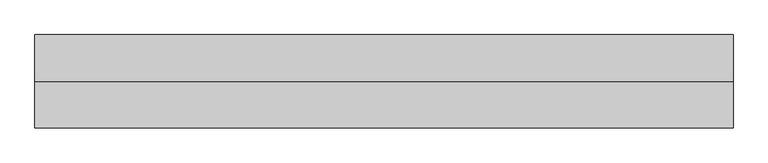
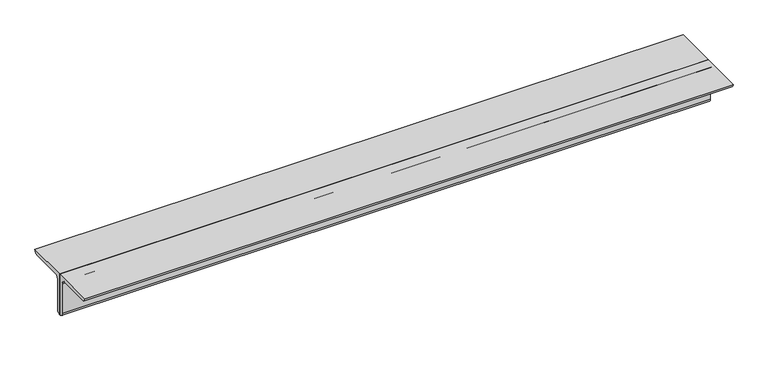
"""IFC4 building model written with IfcOpenShell, lengths in millimetres: member geometry, 0123_Steel Framing_2Ls-KSD3502 : H_SB_AR_S04_2Ls-130x130x12_VBR1."""

from ifc_helpers import new_model, si_unit, point, frame, frame_2d, origin, place, context, project, spatial, polyline, circle_curve, trimmed, segment, composite_curve, outline, extrude, source, transform, mapped, element, save


def member_4cc4f4f8(model_context):
    return source(origin(), model_context, "Body", "SweptSolid", [
        extrude(outline(composite_curve([segment(polyline([(0.0, 36.4), (130.0, 36.4)]), True, "CONTINUOUS"), segment(trimmed(circle_curve(frame_2d((118.0, 36.4)), 12.0), [point((130.0, 36.4))], [point((118.0, 24.4))], False, "CARTESIAN"), True, "CONTINUOUS"), segment(polyline([(118.0, 24.4), (24.0, 24.4)]), True, "CONTINUOUS"), segment(trimmed(circle_curve(frame_2d((24.0, 12.4)), 12.0), [point((24.0, 24.4))], [point((12.0, 12.4))], True, "CARTESIAN"), True, "CONTINUOUS"), segment(polyline([(12.0, 12.4), (12.0, -81.6)]), True, "CONTINUOUS"), segment(trimmed(circle_curve(frame_2d((0.0, -81.6)), 12.0), [point((12.0, -81.6))], [point((0.0, -93.6))], False, "CARTESIAN"), True, "CONTINUOUS"), segment(polyline([(0.0, -93.6), (0.0, 36.4)]), True, "CONTINUOUS")], self_intersect=False)), frame((-905.8182142, 0.0, 0.0), z_axis=(1.0, 0.0, 0.0), x_axis=(0.0, 1.0, 0.0)), (0.0, 0.0, 1.0), 1947.4481229),
        extrude(outline(composite_curve([segment(polyline([(0.0, 36.4), (0.0, -93.6)]), True, "CONTINUOUS"), segment(trimmed(circle_curve(frame_2d((0.0, -81.6)), 12.0), [point((0.0, -93.6))], [point((-12.0, -81.6))], False, "CARTESIAN"), True, "CONTINUOUS"), segment(polyline([(-12.0, -81.6), (-12.0, 12.4)]), True, "CONTINUOUS"), segment(trimmed(circle_curve(frame_2d((-24.0, 12.4)), 12.0), [point((-12.0, 12.4))], [point((-24.0, 24.4))], True, "CARTESIAN"), True, "CONTINUOUS"), segment(polyline([(-24.0, 24.4), (-118.0, 24.4)]), True, "CONTINUOUS"), segment(trimmed(circle_curve(frame_2d((-118.0, 36.4)), 12.0), [point((-118.0, 24.4))], [point((-130.0, 36.4))], False, "CARTESIAN"), True, "CONTINUOUS"), segment(polyline([(-130.0, 36.4), (0.0, 36.4)]), True, "CONTINUOUS")], self_intersect=False)), frame((-905.8182142, 0.0, 0.0), z_axis=(1.0, 0.0, 0.0), x_axis=(0.0, 1.0, 0.0)), (0.0, 0.0, 1.0), 1947.4481229),
    ])


if __name__ == "__main__":
    model = new_model("IFC4")
    model_context = context("Model", 3, world=origin())
    ifc_project = project(units=[si_unit("LENGTHUNIT", "METRE", prefix="MILLI")], contexts=[model_context])
    site = spatial("IfcSite", under=ifc_project)
    building = spatial("IfcBuilding", under=site)
    placement = place(None, origin())
    member_shape = member_4cc4f4f8(model_context)
    element("IfcMember", 1, ObjectType="0123_Steel Framing_2Ls-KSD3502 : H_SB_AR_S04_2Ls-130x130x12_VBR1", at=placement, inside=building, context=model_context, shape_type="MappedRepresentation", body=[
        mapped(member_shape, transform((0.0, 0.0, 0.0), x_axis=(1.0, 0.0, 0.0), y_axis=(0.0, 1.0, 0.0), z_axis=(0.0, 0.0, 1.0))),
    ])
    save(model, "model.ifc")

# Revit data of these elements
# Type "0123_Steel Framing_2Ls-KSD3502 : H_SB_AR_S04_2Ls-130x130x12_VBR1"
#   Assembly Code = "B10"
#   Legs = "SLBB"
#   W = 8.97
#   Perimeter = 1.04 m²/m
#   Nominal Weight = 46.80 kgf/m
#   Length [instance default] = 1000 mm
#   Space = 0 mm
#   b = 130 mm
#   d = 130 mm
#   t = 12 mm
#   y = 36.4 mm
#   A = 0.005952 m²
#   Structural Material [instance default] = Steel ASTM A36
# Element 1 (IfcMember, "0123_Steel Framing_2Ls-KSD3502 : H_SB_AR_S04_2Ls-130x130x12_VBR1")
#   Structural Material = Steel, 45-345
#   Materials on its faces: "Steel, 45-345"
# Materials
#   "Steel ASTM A36": class "Metal", colour RGB 199 199 199, transparency 0, Description = "Structural steel, ASTM A36 Grade B, mill finish", Cost = 0
#   "Steel, 45-345": class "Metal", colour RGB 189 187 185, transparency 0, Description = "Steel 345 MPa", Cost = 0
